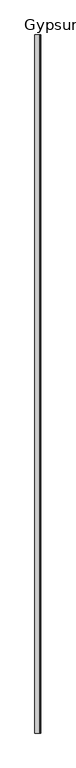
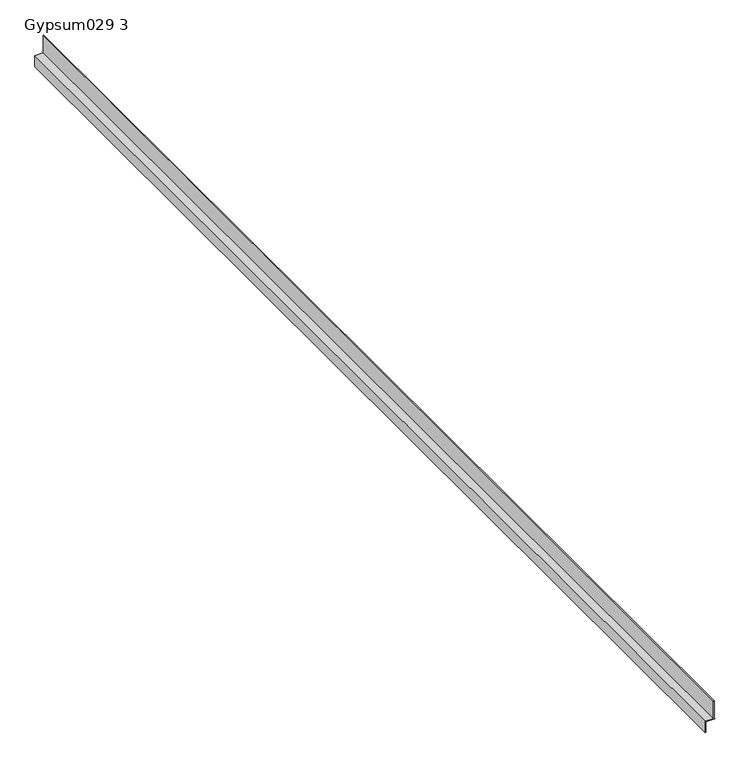
"""IFC4 building model written with IfcOpenShell, lengths in millimetres: proxy geometry, Gypsum029 3 : Gypsum029 6497."""

from ifc_helpers import new_model, si_unit, frame, origin, place, context, project, spatial, polyline, outline, extrude, source, transform, mapped, element, save


def gypsum029_3_ffdc469e(model_context):
    return source(origin(), model_context, "Body", "SweptSolid", [
        extrude(outline(polyline([(36772.596, 10259.6242153), (36791.696, 10259.6242153), (36791.696, 10274.722302), (36792.966, 10274.722302), (36792.966, 10273.9124548), (36824.716, 10273.9124548), (36824.716, 10272.6424548), (36792.966, 10272.6424548), (36792.966, 10258.3542153), (36772.596, 10258.3542153), (36772.596, 10259.6242153)])), frame((0.0, 2217.3610219, 0.0), z_axis=(0.0, 1.0, 0.0), x_axis=(0.0, 0.0, 1.0)), (0.0, 0.0, 1.0), 2000.0),
    ])


if __name__ == "__main__":
    model = new_model("IFC4")
    model_context = context("Model", 3, world=origin())
    ifc_project = project(units=[si_unit("LENGTHUNIT", "METRE", prefix="MILLI")], contexts=[model_context])
    site = spatial("IfcSite", under=ifc_project)
    building = spatial("IfcBuilding", under=site)
    placement = place(None, origin())
    gypsum029_3_shape = gypsum029_3_ffdc469e(model_context)
    element("IfcBuildingElementProxy", 1, Name="Gypsum029 3 : Gypsum029 6497", ObjectType="Gypsum029 3 : Gypsum029 6497", at=placement, inside=building, context=model_context, shape_type="MappedRepresentation", body=[
        mapped(gypsum029_3_shape, transform((0.0, 0.0, 0.0), x_axis=(1.0, 0.0, 0.0), y_axis=(0.0, 1.0, 0.0), z_axis=(0.0, 0.0, 1.0))),
    ])
    save(model, "model.ifc")

# Revit data of these elements
# Type "Gypsum029 3 : Gypsum029 6497"
#   NameOverride = "Gypsum029"
# Element 1 (IfcBuildingElementProxy, "Gypsum029 3 : Gypsum029 6497")
#   Materials on its faces: "SHADOW Z REVEAL  BEAD"
# Materials
#   "SHADOW Z REVEAL  BEAD": class "Unassigned", colour RGB 251 232 155, transparency 0, Cost = 0
